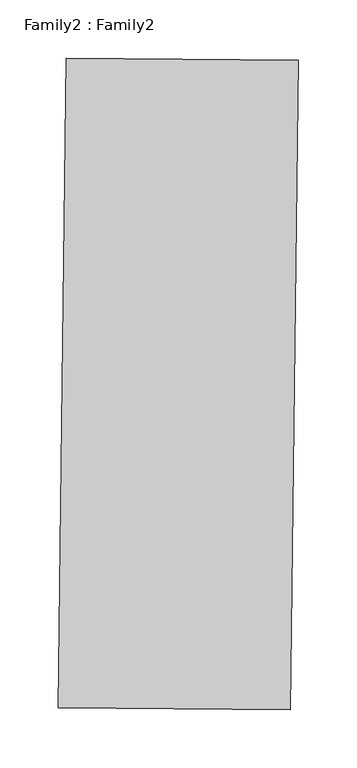
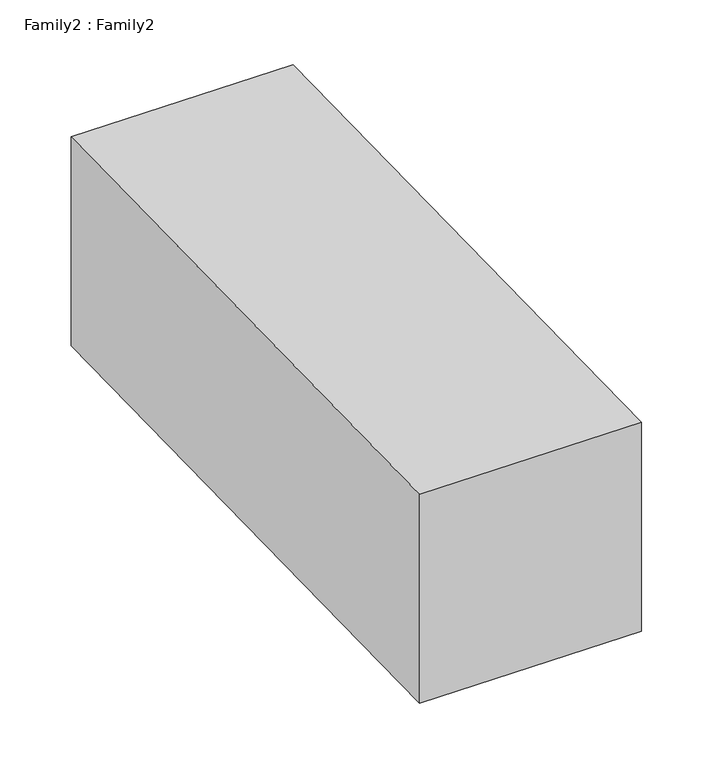
"""IFC4 building model written with IfcOpenShell, lengths in millimetres: proxy geometry, Family2 : Family2."""

import ifcopenshell
import ifcopenshell.guid

model = None  # the IFC model being written
_history = None  # IfcOwnerHistory: only IFC2X3 demands one
_inside = {}  # id of a spatial element -> (the spatial element, [elements in it])
_under = {}  # id of a project, library or spatial element -> (it, [spatial elements below it])
_declared = {}  # id of a project -> (the project, [libraries it declares])
_typed = {}  # id of a type object -> (the type object, [elements of that type])
_made_of = {}  # id of a material, layer set ... -> (it, [elements and type objects made of it])


def new_model(schema):
    """Start an empty IFC model of exactly this schema.

    Asked for "IFC4X3", IfcOpenShell would pick the latest addendum, in which some entities
    have other attributes; the version numbers below select the first issue.
    IFC2X3 requires an IfcOwnerHistory on every rooted entity: one is made here for all.
    """
    global model, _history
    if schema == "IFC4X3":
        model = ifcopenshell.file(schema_version=(4, 3, 0, 0))
    else:
        model = ifcopenshell.file(schema=schema)
    _inside.clear()
    _under.clear()
    _declared.clear()
    _typed.clear()
    _made_of.clear()
    _history = None
    if model.schema == "IFC2X3":
        org = make("IfcOrganization", Name="unknown")
        user = make(
            "IfcPersonAndOrganization",
            ThePerson=make("IfcPerson", FamilyName="unknown"),
            TheOrganization=org,
        )
        app = make(
            "IfcApplication",
            ApplicationDeveloper=org,
            Version="unknown",
            ApplicationFullName="unknown",
            ApplicationIdentifier="unknown",
        )
        _history = make(
            "IfcOwnerHistory",
            OwningUser=user,
            OwningApplication=app,
            ChangeAction="ADDED",
            CreationDate=0,
        )
    return model


def make(cls, **values):
    """One entity of the class cls with the attributes given. An attribute that is None is left unset."""
    return model.create_entity(
        cls, **{name: value for name, value in values.items() if value is not None}
    )


def rooted(cls, **values):
    """An entity with a GlobalId (a new one), such as an element, a storey or a relation."""
    return make(cls, GlobalId=ifcopenshell.guid.new(), OwnerHistory=_history, **values)


def si_unit(unit_type, name, prefix=None):
    """IfcSIUnit, for example si_unit("LENGTHUNIT", "METRE", prefix="MILLI")."""
    return make("IfcSIUnit", UnitType=unit_type, Prefix=prefix, Name=name)


def assignment(units):
    """IfcUnitAssignment: the units of a project."""
    return None if units is None else make("IfcUnitAssignment", Units=units)


def point(xyz):
    """IfcCartesianPoint."""
    return None if xyz is None else make("IfcCartesianPoint", Coordinates=xyz)


def direction(xyz):
    """IfcDirection."""
    return None if xyz is None else make("IfcDirection", DirectionRatios=xyz)


def frame(location, z_axis=None, x_axis=None):
    """IfcAxis2Placement3D, a coordinate frame: its origin and axes. An axis left out is left unset."""
    return make(
        "IfcAxis2Placement3D",
        Location=point(location),
        Axis=direction(z_axis),
        RefDirection=direction(x_axis),
    )


def origin():
    """The frame at (0, 0, 0) with its axes left unset."""
    return frame((0.0, 0.0, 0.0))


def place(relative_to, where):
    """IfcLocalPlacement: puts the frame where relative to a parent placement (None: the world)."""
    return make(
        "IfcLocalPlacement", PlacementRelTo=relative_to, RelativePlacement=where
    )


def context(
    kind, dimensions, precision=None, world=None, true_north=None, identifier=None
):
    """IfcGeometricRepresentationContext, for example the 3D "Model" context."""
    return make(
        "IfcGeometricRepresentationContext",
        ContextIdentifier=identifier,
        ContextType=kind,
        CoordinateSpaceDimension=dimensions,
        Precision=precision,
        WorldCoordinateSystem=world,
        TrueNorth=true_north,
    )


def project(units=None, contexts=None):
    """IfcProject with its units and contexts."""
    return rooted(
        "IfcProject",
        Name="project",
        RepresentationContexts=contexts,
        UnitsInContext=assignment(units),
    )


def spatial(cls, under=None, at=None, **own):
    """A site, building, storey or space (cls), placed at a placement, below another one or the project."""
    s = rooted(cls, ObjectPlacement=at, **own)
    if under is not None:
        _under.setdefault(under.id(), (under, []))[1].append(s)
    return s


def faces_of(points, faces, orient=None, outer=None):
    """IfcFace entities. A face is a list of loops; a loop is a list of indices into points, from 0.

    orient and outer hold one flag for each loop. By default every Orientation is true, the
    first loop of a face is its IfcFaceOuterBound and the others are IfcFaceBound.
    """
    made = []
    for i, loops in enumerate(faces):
        bounds = []
        for j, loop in enumerate(loops):
            is_outer = j == 0 if outer is None else outer[i][j]
            bounds.append(
                make(
                    "IfcFaceOuterBound" if is_outer else "IfcFaceBound",
                    Bound=make("IfcPolyLoop", Polygon=[points[k] for k in loop]),
                    Orientation=True if orient is None else orient[i][j],
                )
            )
        made.append(make("IfcFace", Bounds=bounds))
    return made


def faceted_brep(points, faces, orient=None, outer=None, voids=None):
    """IfcFacetedBrep: a solid bounded by flat faces; with voids (closed shells), ...WithVoids."""
    shared = [point(p) for p in points]
    hull = make("IfcClosedShell", CfsFaces=faces_of(shared, faces, orient, outer))
    if voids is None:
        return make("IfcFacetedBrep", Outer=hull)
    return make(
        "IfcFacetedBrepWithVoids",
        Outer=hull,
        Voids=[
            make(cls, CfsFaces=faces_of(shared, fs, o, b)) for cls, fs, o, b in voids
        ],
    )


def shape(context_of_items, identifier, shape_type, items):
    """IfcShapeRepresentation: the items that make up one representation, for example the "Body"."""
    return make(
        "IfcShapeRepresentation",
        ContextOfItems=context_of_items,
        RepresentationIdentifier=identifier,
        RepresentationType=shape_type,
        Items=items,
    )


def source(mapping_origin, context_of_items, identifier, shape_type, items):
    """IfcRepresentationMap: a shape defined once, which mapped items show again and again."""
    return make(
        "IfcRepresentationMap",
        MappingOrigin=mapping_origin,
        MappedRepresentation=shape(context_of_items, identifier, shape_type, items),
    )


def transform(
    local_origin,
    x_axis=None,
    y_axis=None,
    z_axis=None,
    scale=None,
    scale2=None,
    scale3=None,
    uniform=True,
):
    """IfcCartesianTransformationOperator3D, or its non-uniform kind. x_axis, y_axis, z_axis: its Axis1, 2, 3."""
    if uniform:
        return make(
            "IfcCartesianTransformationOperator3D",
            Axis1=direction(x_axis),
            Axis2=direction(y_axis),
            LocalOrigin=point(local_origin),
            Scale=scale,
            Axis3=direction(z_axis),
        )
    return make(
        "IfcCartesianTransformationOperator3DnonUniform",
        Axis1=direction(x_axis),
        Axis2=direction(y_axis),
        LocalOrigin=point(local_origin),
        Scale=scale,
        Axis3=direction(z_axis),
        Scale2=scale2,
        Scale3=scale3,
    )


def mapped(mapping_source, mapping_target):
    """IfcMappedItem: shows the shape of a source again, moved by a transform."""
    return make(
        "IfcMappedItem", MappingSource=mapping_source, MappingTarget=mapping_target
    )


def made_of(thing, what):
    """Note that an element or type object is made of a material, layer set ...; save() writes the relation."""
    if what is not None:
        _made_of.setdefault(what.id(), (what, []))[1].append(thing)
    return thing


def element(
    cls,
    number,
    at=None,
    inside=None,
    cuts=None,
    type_object=None,
    material=None,
    context=None,
    identifier="Body",
    shape_type=None,
    held_by="IfcProductDefinitionShape",
    body=None,
    shapes=None,
    **own,
):
    """One element of the class cls, such as IfcWall. Its Tag is "e" and its number.

    at: its placement. inside: the storey or other place that contains it. cuts: it is an
    opening in that element (IfcRelVoidsElement). A single representation is given by context,
    identifier, shape_type and body (its items); several are given by shapes. held_by: the class
    of the entity that holds the representations. save() writes the other relations.
    """
    e = rooted(cls, Tag="e%d" % number, ObjectPlacement=at, **own)
    if body is not None:
        shapes = [shape(context, identifier, shape_type, body)]
    if shapes is not None:
        e.Representation = make(held_by, Representations=shapes)
    if inside is not None:
        _inside.setdefault(inside.id(), (inside, []))[1].append(e)
    if cuts is not None:
        rooted(
            "IfcRelVoidsElement", RelatingBuildingElement=cuts, RelatedOpeningElement=e
        )
    if type_object is not None:
        _typed.setdefault(type_object.id(), (type_object, []))[1].append(e)
    return made_of(e, material)


def aggregate(whole, parts):
    """IfcRelAggregates: a whole, such as a stair, and the parts it consists of."""
    return rooted("IfcRelAggregates", RelatingObject=whole, RelatedObjects=parts)


def save(model, path):
    """Write the relations noted so far, then the file.

    IfcRelAggregates (storeys below a building ...), IfcRelContainedInSpatialStructure (elements
    in a storey), IfcRelDefinesByType, IfcRelAssociatesMaterial and IfcRelDeclares: one each for
    every whole, place, type object, material and project.
    """
    for whole, parts in _under.values():
        aggregate(whole, parts)
    for where, things in _inside.values():
        rooted(
            "IfcRelContainedInSpatialStructure",
            RelatedElements=things,
            RelatingStructure=where,
        )
    for kind, things in _typed.values():
        rooted("IfcRelDefinesByType", RelatedObjects=things, RelatingType=kind)
    for what, things in _made_of.values():
        rooted("IfcRelAssociatesMaterial", RelatedObjects=things, RelatingMaterial=what)
    for by, libraries in _declared.values():
        rooted("IfcRelDeclares", RelatingContext=by, RelatedDefinitions=libraries)
    model.write(path)


def family2_family2_b00769dc(model_context):
    return source(origin(), model_context, "Body", "Brep", [
        faceted_brep([(-3946.8595382, -6353.3052302, 1.0945136), (-3946.8595382, -6353.3052302, 201.0945136), (-3939.9832564, -5794.2948924, 202.060409), (-3939.9832564, -5794.2948924, 2.060409), (-3746.8683482, -6355.1824428, 201.0945136), (-3739.9920664, -5796.1721051, 202.060409), (-3746.8683482, -6355.1824428, 1.0945136), (-3739.9920664, -5796.1721051, 2.060409)], [[[0, 1, 2, 3]], [[1, 4, 5, 2]], [[4, 6, 7, 5]], [[6, 0, 3, 7]], [[3, 2, 5, 7]], [[0, 6, 4, 1]]]),
    ])


if __name__ == "__main__":
    model = new_model("IFC4")
    model_context = context("Model", 3, world=origin())
    ifc_project = project(units=[si_unit("LENGTHUNIT", "METRE", prefix="MILLI")], contexts=[model_context])
    site = spatial("IfcSite", under=ifc_project)
    building = spatial("IfcBuilding", under=site)
    placement = place(None, origin())
    family2_family2_shape = family2_family2_b00769dc(model_context)
    element("IfcBuildingElementProxy", 1, Name="Family2 : Family2", ObjectType="Family2 : Family2", at=placement, inside=building, context=model_context, shape_type="MappedRepresentation", body=[
        mapped(family2_family2_shape, transform((0.0, 0.0, 0.0), x_axis=(1.0, 0.0, 0.0), y_axis=(0.0, 1.0, 0.0), z_axis=(0.0, 0.0, 1.0))),
    ])
    save(model, "model.ifc")

# Revit data of these elements
# Type "Family2 : Family2"
#   Default Elevation = 0
